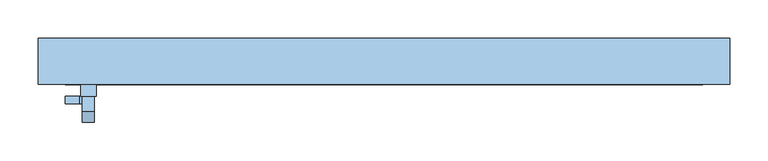
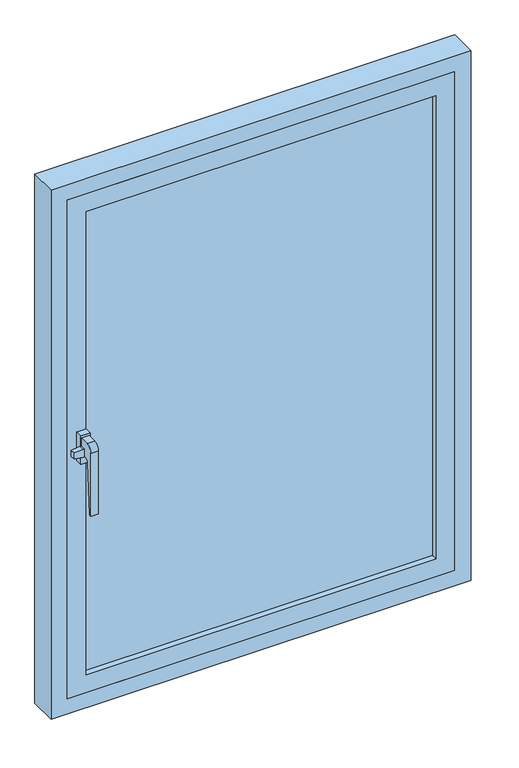
"""IFC4 building model written with IfcOpenShell, lengths in millimetres: window geometry, Inclinar e virar janela - 1 Painel : Inclinar e virar janela - 1 Painel."""

from ifc_helpers import new_model, si_unit, point, frame, frame_2d, origin, place, context, project, spatial, polyline, circle_curve, trimmed, segment, composite_curve, outline, extrude, source, transform, mapped, element, save


def window_efd800ea(model_context):
    return source(origin(), model_context, "Body", "SweptSolid", [
        extrude(outline(composite_curve([segment(polyline([(-95.0, 1259.0), (-95.0, 1241.0), (-100.9630874, 1241.0)]), True, "CONTINUOUS"), segment(trimmed(circle_curve(frame_2d((-100.9630874, 1234.9630874)), 6.0369126), [point((-100.9630874, 1241.0))], [point((-106.9888756, 1235.3294081))], True, "CARTESIAN"), True, "CONTINUOUS"), segment(polyline([(-106.9888756, 1235.3294081), (-114.0, 1120.0), (-119.0, 1120.0), (-119.0, 1263.0)]), True, "CONTINUOUS"), segment(trimmed(circle_curve(frame_2d((-105.0, 1263.0)), 14.0), [point((-119.0, 1263.0))], [point((-105.0, 1277.0))], False, "CARTESIAN"), True, "CONTINUOUS"), segment(polyline([(-105.0, 1277.0), (-85.0, 1277.0), (-85.0, 1259.0), (-95.0, 1259.0)]), True, "CONTINUOUS")], self_intersect=False)), frame((-393.0, 0.0, 0.0), z_axis=(1.0, 0.0, 0.0), x_axis=(0.0, 1.0, 0.0)), (0.0, 0.0, 1.0), 16.0),
        extrude(outline(polyline([(1259.0, -377.0), (1259.0, -396.9864015), (1257.0348924, -415.0), (1243.0157191, -415.0), (1241.0, -396.9864015), (1241.0, -377.0), (1259.0, -377.0)])), frame((0.0, -95.0, 0.0), z_axis=(0.0, 1.0, 0.0), x_axis=(0.0, 0.0, 1.0)), (0.0, 0.0, 1.0), 10.0),
        extrude(outline(polyline([(-395.0, -85.0), (-395.0, -70.0), (-375.0, -70.0), (-375.0, -85.0), (-395.0, -85.0)])), frame((0.0, 0.0, 1218.0), z_axis=(0.0, 0.0, 1.0), x_axis=(1.0, 0.0, 0.0)), (0.0, 0.0, 1.0), 64.0),
        extrude(outline(polyline([(375.0, -43.0), (375.0, -57.0), (-375.0, -57.0), (-375.0, -43.0), (375.0, -43.0)])), frame((0.0, 0.0, 725.0), z_axis=(0.0, 0.0, 1.0), x_axis=(1.0, 0.0, 0.0)), (0.0, 0.0, 1.0), 1050.0),
        extrude(outline(polyline([(685.0, -415.0), (685.0, 415.0), (1815.0, 415.0), (1815.0, -415.0), (685.0, -415.0)]), holes=[polyline([(1775.0, -375.0), (1775.0, 375.0), (725.0, 375.0), (725.0, -375.0), (1775.0, -375.0)])]), frame((0.0, -70.0, 0.0), z_axis=(0.0, 1.0, 0.0), x_axis=(0.0, 0.0, 1.0)), (0.0, 0.0, 1.0), 40.0),
        extrude(outline(polyline([(650.0, -450.0), (650.0, 450.0), (1850.0, 450.0), (1850.0, -450.0), (650.0, -450.0)]), holes=[polyline([(1815.0, -415.0), (1815.0, 415.0), (685.0, 415.0), (685.0, -415.0), (1815.0, -415.0)])]), frame((0.0, -70.0, 0.0), z_axis=(0.0, 1.0, 0.0), x_axis=(0.0, 0.0, 1.0)), (0.0, 0.0, 1.0), 60.0),
    ])


if __name__ == "__main__":
    model = new_model("IFC4")
    model_context = context("Model", 3, world=origin())
    ifc_project = project(units=[si_unit("LENGTHUNIT", "METRE", prefix="MILLI")], contexts=[model_context])
    site = spatial("IfcSite", under=ifc_project)
    building = spatial("IfcBuilding", under=site)
    placement = place(None, origin())
    window_shape = window_efd800ea(model_context)
    element("IfcWindow", 1, ObjectType="Inclinar e virar janela - 1 Painel : Inclinar e virar janela - 1 Painel", at=placement, inside=building, context=model_context, shape_type="MappedRepresentation", body=[
        mapped(window_shape, transform((0.0, 0.0, 0.0), x_axis=(1.0, 0.0, 0.0), y_axis=(0.0, 1.0, 0.0), z_axis=(0.0, 0.0, 1.0))),
    ])
    save(model, "model.ifc")

# Revit data of these elements
# Type "Inclinar e virar janela - 1 Painel : Inclinar e virar janela - 1 Painel"
#   Type Mark = "EF28"
#   Construction Type Id = "SGL"
#   Analytic Construction = "Janelas grandes envidraçadas únicas"
#   W1 = 0.830 m
#   Visual Light Transmittance = 0.9
#   Solar Heat Gain Coefficient = 0.86
#   Rough Width = 0.900 m
#   Rough Height = 1.200 m
#   Largura da moldura do painel = 0.040 m
#   Espessura da moldura do painel = 0.040 m
#   Height = 1.200 m
#   Heat Transfer Coefficient (U) = 5.5617 W/(m²·K)
#   H1 = 1.130 m
#   Largura da estrutura = 0.035 m
#   Espessura da moldura = 0.060 m
#   Altura-padrão do peitoril = 0.650 m
#   Width = 0.900 m
#   Define Thermal Properties by = 1
#   Material do puxador = none
#   Vidro = none
#   Material da moldura = none
#   Wall Closure = (empty or 0)
# Element 1 (IfcWindow, "Inclinar e virar janela - 1 Painel : Inclinar e virar janela - 1 Painel")
#   Materials on its faces: "Glass"
# Materials
#   "Glass": class "Glass", colour RGB 0 128 192, transparency 0.75, Description = "Soda Lime Glass", Cost = 0
